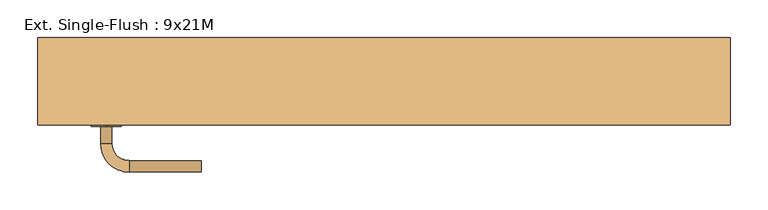
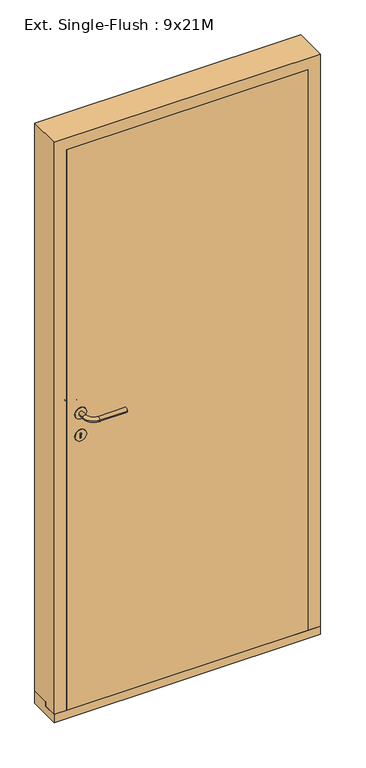
"""IFC4 building model written with IfcOpenShell, lengths in millimetres: door geometry, Ext. Single-Flush : 9x21M."""

import ifcopenshell
import ifcopenshell.guid

model = None  # the IFC model being written
_history = None  # IfcOwnerHistory: only IFC2X3 demands one
_inside = {}  # id of a spatial element -> (the spatial element, [elements in it])
_under = {}  # id of a project, library or spatial element -> (it, [spatial elements below it])
_declared = {}  # id of a project -> (the project, [libraries it declares])
_typed = {}  # id of a type object -> (the type object, [elements of that type])
_made_of = {}  # id of a material, layer set ... -> (it, [elements and type objects made of it])


def new_model(schema):
    """Start an empty IFC model of exactly this schema.

    Asked for "IFC4X3", IfcOpenShell would pick the latest addendum, in which some entities
    have other attributes; the version numbers below select the first issue.
    IFC2X3 requires an IfcOwnerHistory on every rooted entity: one is made here for all.
    """
    global model, _history
    if schema == "IFC4X3":
        model = ifcopenshell.file(schema_version=(4, 3, 0, 0))
    else:
        model = ifcopenshell.file(schema=schema)
    _inside.clear()
    _under.clear()
    _declared.clear()
    _typed.clear()
    _made_of.clear()
    _history = None
    if model.schema == "IFC2X3":
        org = make("IfcOrganization", Name="unknown")
        user = make(
            "IfcPersonAndOrganization",
            ThePerson=make("IfcPerson", FamilyName="unknown"),
            TheOrganization=org,
        )
        app = make(
            "IfcApplication",
            ApplicationDeveloper=org,
            Version="unknown",
            ApplicationFullName="unknown",
            ApplicationIdentifier="unknown",
        )
        _history = make(
            "IfcOwnerHistory",
            OwningUser=user,
            OwningApplication=app,
            ChangeAction="ADDED",
            CreationDate=0,
        )
    return model


def make(cls, **values):
    """One entity of the class cls with the attributes given. An attribute that is None is left unset."""
    return model.create_entity(
        cls, **{name: value for name, value in values.items() if value is not None}
    )


def rooted(cls, **values):
    """An entity with a GlobalId (a new one), such as an element, a storey or a relation."""
    return make(cls, GlobalId=ifcopenshell.guid.new(), OwnerHistory=_history, **values)


def si_unit(unit_type, name, prefix=None):
    """IfcSIUnit, for example si_unit("LENGTHUNIT", "METRE", prefix="MILLI")."""
    return make("IfcSIUnit", UnitType=unit_type, Prefix=prefix, Name=name)


def assignment(units):
    """IfcUnitAssignment: the units of a project."""
    return None if units is None else make("IfcUnitAssignment", Units=units)


def point(xyz):
    """IfcCartesianPoint."""
    return None if xyz is None else make("IfcCartesianPoint", Coordinates=xyz)


def direction(xyz):
    """IfcDirection."""
    return None if xyz is None else make("IfcDirection", DirectionRatios=xyz)


def frame(location, z_axis=None, x_axis=None):
    """IfcAxis2Placement3D, a coordinate frame: its origin and axes. An axis left out is left unset."""
    return make(
        "IfcAxis2Placement3D",
        Location=point(location),
        Axis=direction(z_axis),
        RefDirection=direction(x_axis),
    )


def frame_2d(location, x_axis=None):
    """IfcAxis2Placement2D, a coordinate frame in the plane: its origin and x axis."""
    return make(
        "IfcAxis2Placement2D", Location=point(location), RefDirection=direction(x_axis)
    )


def origin():
    """The frame at (0, 0, 0) with its axes left unset."""
    return frame((0.0, 0.0, 0.0))


def place(relative_to, where):
    """IfcLocalPlacement: puts the frame where relative to a parent placement (None: the world)."""
    return make(
        "IfcLocalPlacement", PlacementRelTo=relative_to, RelativePlacement=where
    )


def context(
    kind, dimensions, precision=None, world=None, true_north=None, identifier=None
):
    """IfcGeometricRepresentationContext, for example the 3D "Model" context."""
    return make(
        "IfcGeometricRepresentationContext",
        ContextIdentifier=identifier,
        ContextType=kind,
        CoordinateSpaceDimension=dimensions,
        Precision=precision,
        WorldCoordinateSystem=world,
        TrueNorth=true_north,
    )


def project(units=None, contexts=None):
    """IfcProject with its units and contexts."""
    return rooted(
        "IfcProject",
        Name="project",
        RepresentationContexts=contexts,
        UnitsInContext=assignment(units),
    )


def spatial(cls, under=None, at=None, **own):
    """A site, building, storey or space (cls), placed at a placement, below another one or the project."""
    s = rooted(cls, ObjectPlacement=at, **own)
    if under is not None:
        _under.setdefault(under.id(), (under, []))[1].append(s)
    return s


def polyline(points):
    """IfcPolyline through the points."""
    return make("IfcPolyline", Points=[point(p) for p in points])


def circle_curve(where, radius):
    """IfcCircle in the frame where."""
    return make("IfcCircle", Position=where, Radius=radius)


def ellipse_curve(where, semi_axis1, semi_axis2):
    """IfcEllipse in the frame where."""
    return make(
        "IfcEllipse", Position=where, SemiAxis1=semi_axis1, SemiAxis2=semi_axis2
    )


def trimmed(basis, trim1, trim2, sense, master):
    """IfcTrimmedCurve: the piece of a basis curve between two trims."""
    return make(
        "IfcTrimmedCurve",
        BasisCurve=basis,
        Trim1=trim1,
        Trim2=trim2,
        SenseAgreement=sense,
        MasterRepresentation=master,
    )


def segment(curve, same_sense, transition):
    """IfcCompositeCurveSegment."""
    return make(
        "IfcCompositeCurveSegment",
        Transition=transition,
        SameSense=same_sense,
        ParentCurve=curve,
    )


def composite_curve(segments, self_intersect=None):
    """IfcCompositeCurve: segments joined end to end."""
    return make("IfcCompositeCurve", Segments=segments, SelfIntersect=self_intersect)


def outline(outer, holes=None, kind="AREA"):
    """IfcArbitraryClosedProfileDef: a profile drawn as a closed curve; with holes, ...WithVoids."""
    if holes is None:
        return make("IfcArbitraryClosedProfileDef", ProfileType=kind, OuterCurve=outer)
    return make(
        "IfcArbitraryProfileDefWithVoids",
        ProfileType=kind,
        OuterCurve=outer,
        InnerCurves=holes,
    )


def extrude(swept, where, along, depth):
    """IfcExtrudedAreaSolid: the profile swept, set in the frame where, extruded along a direction by depth."""
    return make(
        "IfcExtrudedAreaSolid",
        SweptArea=swept,
        Position=where,
        ExtrudedDirection=direction(along),
        Depth=depth,
    )


def faces_of(points, faces, orient=None, outer=None):
    """IfcFace entities. A face is a list of loops; a loop is a list of indices into points, from 0.

    orient and outer hold one flag for each loop. By default every Orientation is true, the
    first loop of a face is its IfcFaceOuterBound and the others are IfcFaceBound.
    """
    made = []
    for i, loops in enumerate(faces):
        bounds = []
        for j, loop in enumerate(loops):
            is_outer = j == 0 if outer is None else outer[i][j]
            bounds.append(
                make(
                    "IfcFaceOuterBound" if is_outer else "IfcFaceBound",
                    Bound=make("IfcPolyLoop", Polygon=[points[k] for k in loop]),
                    Orientation=True if orient is None else orient[i][j],
                )
            )
        made.append(make("IfcFace", Bounds=bounds))
    return made


def faceted_brep(points, faces, orient=None, outer=None, voids=None):
    """IfcFacetedBrep: a solid bounded by flat faces; with voids (closed shells), ...WithVoids."""
    shared = [point(p) for p in points]
    hull = make("IfcClosedShell", CfsFaces=faces_of(shared, faces, orient, outer))
    if voids is None:
        return make("IfcFacetedBrep", Outer=hull)
    return make(
        "IfcFacetedBrepWithVoids",
        Outer=hull,
        Voids=[
            make(cls, CfsFaces=faces_of(shared, fs, o, b)) for cls, fs, o, b in voids
        ],
    )


def shape(context_of_items, identifier, shape_type, items):
    """IfcShapeRepresentation: the items that make up one representation, for example the "Body"."""
    return make(
        "IfcShapeRepresentation",
        ContextOfItems=context_of_items,
        RepresentationIdentifier=identifier,
        RepresentationType=shape_type,
        Items=items,
    )


def source(mapping_origin, context_of_items, identifier, shape_type, items):
    """IfcRepresentationMap: a shape defined once, which mapped items show again and again."""
    return make(
        "IfcRepresentationMap",
        MappingOrigin=mapping_origin,
        MappedRepresentation=shape(context_of_items, identifier, shape_type, items),
    )


def transform(
    local_origin,
    x_axis=None,
    y_axis=None,
    z_axis=None,
    scale=None,
    scale2=None,
    scale3=None,
    uniform=True,
):
    """IfcCartesianTransformationOperator3D, or its non-uniform kind. x_axis, y_axis, z_axis: its Axis1, 2, 3."""
    if uniform:
        return make(
            "IfcCartesianTransformationOperator3D",
            Axis1=direction(x_axis),
            Axis2=direction(y_axis),
            LocalOrigin=point(local_origin),
            Scale=scale,
            Axis3=direction(z_axis),
        )
    return make(
        "IfcCartesianTransformationOperator3DnonUniform",
        Axis1=direction(x_axis),
        Axis2=direction(y_axis),
        LocalOrigin=point(local_origin),
        Scale=scale,
        Axis3=direction(z_axis),
        Scale2=scale2,
        Scale3=scale3,
    )


def mapped(mapping_source, mapping_target):
    """IfcMappedItem: shows the shape of a source again, moved by a transform."""
    return make(
        "IfcMappedItem", MappingSource=mapping_source, MappingTarget=mapping_target
    )


def made_of(thing, what):
    """Note that an element or type object is made of a material, layer set ...; save() writes the relation."""
    if what is not None:
        _made_of.setdefault(what.id(), (what, []))[1].append(thing)
    return thing


def element(
    cls,
    number,
    at=None,
    inside=None,
    cuts=None,
    type_object=None,
    material=None,
    context=None,
    identifier="Body",
    shape_type=None,
    held_by="IfcProductDefinitionShape",
    body=None,
    shapes=None,
    **own,
):
    """One element of the class cls, such as IfcWall. Its Tag is "e" and its number.

    at: its placement. inside: the storey or other place that contains it. cuts: it is an
    opening in that element (IfcRelVoidsElement). A single representation is given by context,
    identifier, shape_type and body (its items); several are given by shapes. held_by: the class
    of the entity that holds the representations. save() writes the other relations.
    """
    e = rooted(cls, Tag="e%d" % number, ObjectPlacement=at, **own)
    if body is not None:
        shapes = [shape(context, identifier, shape_type, body)]
    if shapes is not None:
        e.Representation = make(held_by, Representations=shapes)
    if inside is not None:
        _inside.setdefault(inside.id(), (inside, []))[1].append(e)
    if cuts is not None:
        rooted(
            "IfcRelVoidsElement", RelatingBuildingElement=cuts, RelatedOpeningElement=e
        )
    if type_object is not None:
        _typed.setdefault(type_object.id(), (type_object, []))[1].append(e)
    return made_of(e, material)


def aggregate(whole, parts):
    """IfcRelAggregates: a whole, such as a stair, and the parts it consists of."""
    return rooted("IfcRelAggregates", RelatingObject=whole, RelatedObjects=parts)


def save(model, path):
    """Write the relations noted so far, then the file.

    IfcRelAggregates (storeys below a building ...), IfcRelContainedInSpatialStructure (elements
    in a storey), IfcRelDefinesByType, IfcRelAssociatesMaterial and IfcRelDeclares: one each for
    every whole, place, type object, material and project.
    """
    for whole, parts in _under.values():
        aggregate(whole, parts)
    for where, things in _inside.values():
        rooted(
            "IfcRelContainedInSpatialStructure",
            RelatedElements=things,
            RelatingStructure=where,
        )
    for kind, things in _typed.values():
        rooted("IfcRelDefinesByType", RelatedObjects=things, RelatingType=kind)
    for what, things in _made_of.values():
        rooted("IfcRelAssociatesMaterial", RelatedObjects=things, RelatingMaterial=what)
    for by, libraries in _declared.values():
        rooted("IfcRelDeclares", RelatingContext=by, RelatedDefinitions=libraries)
    model.write(path)


def plane_surface(at):
    """IfcPlane: the flat surface through the origin of the frame at, square to its z axis."""
    return make("IfcPlane", Position=at)


def cylinder_surface(at, radius):
    """IfcCylindricalSurface: all points at the distance radius from the z axis of the frame at."""
    return make("IfcCylindricalSurface", Position=at, Radius=radius)


def revolved_surface(curve, axis_point, axis_direction):
    """IfcSurfaceOfRevolution: the curve turned about the line through axis_point along axis_direction."""
    return make(
        "IfcSurfaceOfRevolution",
        SweptCurve=make("IfcArbitraryOpenProfileDef", ProfileType="CURVE", Curve=curve),
        AxisPosition=make("IfcAxis1Placement", Location=point(axis_point), Axis=direction(axis_direction)),
    )


def advanced_brep(points, edges, surfaces, faces):
    """IfcAdvancedBrep: a solid bounded by faces that lie on surfaces and meet in shared edges.

    An edge is (start, end): straight between two places in points (the first is 0);
    or (start, end, curve); or (start, end, curve, False) where it runs against its curve.
    A face is (place in surfaces, loops), or (place, loops, False) where it looks against
    its surface's normal. A loop lists edges by number (the first is 1), with a minus sign
    where the edge is run from its end to its start. The first loop is the outer one.
    """
    corners = [point(p) for p in points]
    vertices = [make("IfcVertexPoint", VertexGeometry=c) for c in corners]
    made = []
    for start, end, *more in edges:
        made.append(
            make(
                "IfcEdgeCurve",
                EdgeStart=vertices[start],
                EdgeEnd=vertices[end],
                EdgeGeometry=more[0] if more else make("IfcPolyline", Points=[corners[start], corners[end]]),
                SameSense=more[1] if len(more) > 1 else True,
            )
        )
    hull = []
    for where, loops, *sense in faces:
        bounds = []
        for j, loop in enumerate(loops):
            ring = [make("IfcOrientedEdge", EdgeElement=made[abs(k) - 1], Orientation=k > 0) for k in loop]
            bounds.append(
                make(
                    "IfcFaceOuterBound" if j == 0 else "IfcFaceBound",
                    Bound=make("IfcEdgeLoop", EdgeList=ring),
                    Orientation=True,
                )
            )
        hull.append(make("IfcAdvancedFace", Bounds=bounds, FaceSurface=surfaces[where], SameSense=sense[0] if sense else True))
    return make("IfcAdvancedBrep", Outer=make("IfcClosedShell", CfsFaces=hull))


def ext_single_flush_9x21m_ea871c4f(model_context):
    return source(origin(), model_context, "Body", "SolidModel", [
        extrude(outline(composite_curve([segment(trimmed(circle_curve(frame_2d((1090.0, -366.0)), 20.0), [point((1070.0, -366.0))], [point((1110.0, -366.0))], False, "CARTESIAN"), True, "CONTINUOUS"), segment(trimmed(circle_curve(frame_2d((1090.0, -366.0)), 20.0), [point((1110.0, -366.0))], [point((1070.0, -366.0))], False, "CARTESIAN"), True, "CONTINUOUS")], self_intersect=False)), frame((0.0, -186.0, 0.0), z_axis=(0.0, 1.0, 0.0), x_axis=(0.0, 0.0, 1.0)), (0.0, 0.0, 1.0), 2.0),
        advanced_brep(
        [(-373.5, -186.0, 1090.0), (-358.5, -186.0, 1090.0), (-358.5, -208.5, 1090.0), (-373.5, -208.5, 1090.0), (-336.0, -231.0, 1090.0), (-336.0, -246.0, 1090.0), (-241.0, -231.0, 1090.0), (-241.0, -246.0, 1090.0)],
        [
            (0, 1, circle_curve(frame((-366.0, -186.0, 1090.0), z_axis=(0.0, 1.0, 0.0), x_axis=(1.0, 0.0, 0.0)), 7.5)),
            (1, 0, circle_curve(frame((-366.0, -186.0, 1090.0), z_axis=(0.0, 1.0, 0.0), x_axis=(1.0, 0.0, 0.0)), 7.5)),
            (1, 2),
            (2, 3, circle_curve(frame((-366.0, -208.5, 1090.0), z_axis=(0.0, 1.0, 0.0), x_axis=(1.0, 0.0, 0.0)), 7.5)),
            (3, 0),
            (3, 2, circle_curve(frame((-366.0, -208.5, 1090.0), z_axis=(0.0, 1.0, 0.0), x_axis=(1.0, 0.0, 0.0)), 7.5)),
            (4, 5, circle_curve(frame((-336.0, -238.5, 1090.0), z_axis=(-1.0, 0.0, 0.0), x_axis=(0.0, 1.0, 0.0)), 7.5)),
            (5, 3, circle_curve(frame((-336.0, -208.5, 1090.0), z_axis=(0.0, 0.0, -1.0), x_axis=(-1.0, 0.0, 0.0)), 37.5)),
            (2, 4, circle_curve(frame((-336.0, -208.5, 1090.0), z_axis=(0.0, 0.0, 1.0), x_axis=(-1.0, 0.0, 0.0)), 22.5)),
            (5, 4, circle_curve(frame((-336.0, -238.5, 1090.0), z_axis=(-1.0, 0.0, 0.0), x_axis=(0.0, 1.0, 0.0)), 7.5)),
            (4, 6),
            (6, 7, circle_curve(frame((-241.0, -238.5, 1090.0), z_axis=(-1.0, 0.0, 0.0), x_axis=(0.0, 1.0, 0.0)), 7.5)),
            (7, 5),
            (7, 6, circle_curve(frame((-241.0, -238.5, 1090.0), z_axis=(-1.0, 0.0, 0.0), x_axis=(0.0, 1.0, 0.0)), 7.5)),
        ],
        [
            plane_surface(frame((-366.0, -186.0, 1090.0), z_axis=(0.0, 1.0, 0.0), x_axis=(0.0, 0.0, -1.0))),
            cylinder_surface(frame((-366.0, -186.0, 1090.0), z_axis=(0.0, 1.0, 0.0), x_axis=(1.0, 0.0, 0.0)), 7.5),
            revolved_surface(trimmed(ellipse_curve(frame((-366.0, -208.5, 1090.0), z_axis=(0.0, -1.0, 0.0), x_axis=(1.0, 0.0, 0.0)), 7.5, 7.5), [point((-373.5, -208.5, 1090.0))], [point((-358.5, -208.5, 1090.0))], True, "CARTESIAN"), (-336.0, -208.5, 1090.0), (0.0, 0.0, -1.0)),
            revolved_surface(trimmed(ellipse_curve(frame((-366.0, -208.5, 1090.0), z_axis=(0.0, -1.0, 0.0), x_axis=(1.0, 0.0, 0.0)), 7.5, 7.5), [point((-358.5, -208.5, 1090.0))], [point((-373.5, -208.5, 1090.0))], True, "CARTESIAN"), (-336.0, -208.5, 1090.0), (0.0, 0.0, -1.0)),
            cylinder_surface(frame((-336.0, -238.5, 1090.0), z_axis=(-1.0, 0.0, 0.0), x_axis=(0.0, 1.0, 0.0)), 7.5),
            plane_surface(frame((-241.0, -238.5, 1090.0), z_axis=(1.0, 0.0, 0.0), x_axis=(0.0, 0.0, -1.0))),
        ],
        [
            (0, [[1, 2]]),
            (1, [[3, 4, 5, -2]]),
            (1, [[-5, 6, -3, -1]]),
            (2, [[7, 8, -4, 9]]),
            (3, [[10, -9, -6, -8]]),
            (4, [[11, 12, 13, -7]]),
            (4, [[-13, 14, -11, -10]]),
            (5, [[-12, -14]]),
        ],
    ),
        extrude(outline(composite_curve([segment(trimmed(circle_curve(frame_2d((1010.0, -366.0)), 20.0), [point((990.0, -366.0))], [point((1030.0, -366.0))], False, "CARTESIAN"), True, "CONTINUOUS"), segment(trimmed(circle_curve(frame_2d((1010.0, -366.0)), 20.0), [point((1030.0, -366.0))], [point((990.0, -366.0))], False, "CARTESIAN"), True, "CONTINUOUS")], self_intersect=False), holes=[composite_curve([segment(trimmed(circle_curve(frame_2d((1015.0, -366.0)), 3.0), [point((1012.4019238, -367.5))], [point((1012.4019238, -364.5))], True, "CARTESIAN"), True, "CONTINUOUS"), segment(polyline([(1012.4019238, -364.5), (1000.0, -364.5), (1000.0, -367.5), (1012.4019238, -367.5)]), True, "CONTINUOUS")], self_intersect=False)]), frame((0.0, -186.0, 0.0), z_axis=(0.0, 1.0, 0.0), x_axis=(0.0, 0.0, 1.0)), (0.0, 0.0, 1.0), 2.0),
        extrude(outline(composite_curve([segment(trimmed(circle_curve(frame_2d((1090.0, -366.0)), 20.0), [point((1070.0, -366.0))], [point((1110.0, -366.0))], False, "CARTESIAN"), True, "CONTINUOUS"), segment(trimmed(circle_curve(frame_2d((1090.0, -366.0)), 20.0), [point((1110.0, -366.0))], [point((1070.0, -366.0))], False, "CARTESIAN"), True, "CONTINUOUS")], self_intersect=False)), frame((0.0, -134.0, 0.0), z_axis=(0.0, 1.0, 0.0), x_axis=(0.0, 0.0, 1.0)), (0.0, 0.0, 1.0), 2.0),
        advanced_brep(
        [(-373.5, -132.0, 1090.0), (-358.5, -132.0, 1090.0), (-373.5, -109.5, 1090.0), (-358.5, -109.5, 1090.0), (-336.0, -87.0, 1090.0), (-336.0, -72.0, 1090.0), (-241.0, -72.0, 1090.0), (-241.0, -87.0, 1090.0)],
        [
            (0, 1, circle_curve(frame((-366.0, -132.0, 1090.0), z_axis=(0.0, -1.0, 0.0), x_axis=(1.0, 0.0, 0.0)), 7.5)),
            (1, 0, circle_curve(frame((-366.0, -132.0, 1090.0), z_axis=(0.0, -1.0, 0.0), x_axis=(1.0, 0.0, 0.0)), 7.5)),
            (0, 2),
            (2, 3, circle_curve(frame((-366.0, -109.5, 1090.0), z_axis=(0.0, -1.0, 0.0), x_axis=(1.0, 0.0, 0.0)), 7.5)),
            (3, 1),
            (3, 2, circle_curve(frame((-366.0, -109.5, 1090.0), z_axis=(0.0, -1.0, 0.0), x_axis=(1.0, 0.0, 0.0)), 7.5)),
            (4, 3, circle_curve(frame((-336.0, -109.5, 1090.0), z_axis=(0.0, 0.0, 1.0), x_axis=(-1.0, 0.0, 0.0)), 22.5)),
            (2, 5, circle_curve(frame((-336.0, -109.5, 1090.0), z_axis=(0.0, 0.0, -1.0), x_axis=(-1.0, 0.0, 0.0)), 37.5)),
            (5, 4, circle_curve(frame((-336.0, -79.5, 1090.0), z_axis=(-1.0, 0.0, 0.0), x_axis=(0.0, -1.0, 0.0)), 7.5)),
            (4, 5, circle_curve(frame((-336.0, -79.5, 1090.0), z_axis=(-1.0, 0.0, 0.0), x_axis=(0.0, -1.0, 0.0)), 7.5)),
            (5, 6),
            (6, 7, circle_curve(frame((-241.0, -79.5, 1090.0), z_axis=(-1.0, 0.0, 0.0), x_axis=(0.0, -1.0, 0.0)), 7.5)),
            (7, 4),
            (7, 6, circle_curve(frame((-241.0, -79.5, 1090.0), z_axis=(-1.0, 0.0, 0.0), x_axis=(0.0, -1.0, 0.0)), 7.5)),
        ],
        [
            plane_surface(frame((-366.0, -132.0, 1090.0), z_axis=(0.0, -1.0, 0.0), x_axis=(0.0, 0.0, -1.0))),
            cylinder_surface(frame((-366.0, -132.0, 1090.0), z_axis=(0.0, -1.0, 0.0), x_axis=(1.0, 0.0, 0.0)), 7.5),
            revolved_surface(trimmed(ellipse_curve(frame((-366.0, -109.5, 1090.0), z_axis=(0.0, -1.0, 0.0), x_axis=(1.0, 0.0, 0.0)), 7.5, 7.5), [point((-373.5, -109.5, 1090.0))], [point((-358.5, -109.5, 1090.0))], True, "CARTESIAN"), (-336.0, -109.5, 1090.0), (0.0, 0.0, -1.0)),
            revolved_surface(trimmed(ellipse_curve(frame((-366.0, -109.5, 1090.0), z_axis=(0.0, -1.0, 0.0), x_axis=(1.0, 0.0, 0.0)), 7.5, 7.5), [point((-358.5, -109.5, 1090.0))], [point((-373.5, -109.5, 1090.0))], True, "CARTESIAN"), (-336.0, -109.5, 1090.0), (0.0, 0.0, -1.0)),
            cylinder_surface(frame((-336.0, -79.5, 1090.0), z_axis=(-1.0, 0.0, 0.0), x_axis=(0.0, -1.0, 0.0)), 7.5),
            plane_surface(frame((-241.0, -79.5, 1090.0), z_axis=(1.0, 0.0, 0.0), x_axis=(0.0, 0.0, -1.0))),
        ],
        [
            (0, [[1, 2]]),
            (1, [[-1, 3, 4, 5]]),
            (1, [[-2, -5, 6, -3]]),
            (2, [[7, -4, 8, 9]]),
            (3, [[-8, -6, -7, 10]]),
            (4, [[-9, 11, 12, 13]]),
            (4, [[-10, -13, 14, -11]]),
            (5, [[-14, -12]]),
        ],
    ),
        extrude(outline(composite_curve([segment(trimmed(circle_curve(frame_2d((1010.0, -366.0)), 20.0), [point((990.0, -366.0))], [point((1030.0, -366.0))], False, "CARTESIAN"), True, "CONTINUOUS"), segment(trimmed(circle_curve(frame_2d((1010.0, -366.0)), 20.0), [point((1030.0, -366.0))], [point((990.0, -366.0))], False, "CARTESIAN"), True, "CONTINUOUS")], self_intersect=False), holes=[composite_curve([segment(trimmed(circle_curve(frame_2d((1015.0, -366.0)), 3.0), [point((1012.4019238, -367.5))], [point((1012.4019238, -364.5))], True, "CARTESIAN"), True, "CONTINUOUS"), segment(polyline([(1012.4019238, -364.5), (1000.0, -364.5), (1000.0, -367.5), (1012.4019238, -367.5)]), True, "CONTINUOUS")], self_intersect=False)]), frame((0.0, -134.0, 0.0), z_axis=(0.0, 1.0, 0.0), x_axis=(0.0, 0.0, 1.0)), (0.0, 0.0, 1.0), 2.0),
        extrude(outline(polyline([(-414.0, -184.0), (-414.0, -134.0), (414.0, -134.0), (414.0, -184.0), (-414.0, -184.0)])), frame((0.0, 0.0, 30.0), z_axis=(0.0, 0.0, 1.0), x_axis=(1.0, 0.0, 0.0)), (0.0, 0.0, 1.0), 2028.0),
        faceted_brep([(414.0, -184.0, 2058.0), (414.0, -184.0, 30.0), (456.0, -184.0, 30.0), (456.0, -184.0, 2100.0), (-456.0, -184.0, 2100.0), (-456.0, -184.0, 30.0), (-414.0, -184.0, 30.0), (-414.0, -184.0, 2058.0), (-414.0, -134.0, 30.0), (-414.0, -134.0, 45.0), (-414.0, -134.0, 2058.0), (-456.0, -134.0, 30.0), (456.0, -134.0, 30.0), (414.0, -134.0, 30.0), (-456.0, -69.0, 2100.0), (-456.0, -69.0, 45.0), (-456.0, -134.0, 45.0), (456.0, -134.0, 45.0), (456.0, -69.0, 45.0), (456.0, -69.0, 2100.0), (414.0, -134.0, 2058.0), (414.0, -134.0, 45.0), (399.0, -69.0, 45.0), (399.0, -69.0, 2043.0), (-399.0, -69.0, 2043.0), (-399.0, -69.0, 45.0), (-399.0, -134.0, 45.0), (399.0, -134.0, 45.0), (-399.0, -134.0, 2043.0), (399.0, -134.0, 2043.0)], [[[0, 1, 2, 3, 4, 5, 6, 7]], [[7, 6, 8, 9, 10]], [[8, 6, 5, 11]], [[12, 2, 1, 13]], [[14, 15, 16, 11, 5, 4]], [[3, 2, 12, 17, 18, 19]], [[20, 21, 13, 1, 0]], [[19, 18, 22, 23, 24, 25, 15, 14]], [[16, 15, 25, 26, 9]], [[21, 27, 22, 18, 17]], [[9, 8, 11, 16]], [[17, 12, 13, 21]], [[28, 26, 25, 24]], [[23, 22, 27, 29]], [[29, 27, 21, 20, 10, 9, 26, 28]], [[3, 19, 14, 4]], [[23, 29, 28, 24]], [[7, 10, 20, 0]]]),
        extrude(outline(polyline([(-184.0, 30.0), (-134.0, 30.0), (-134.0, 45.0), (-69.0, 45.0), (-69.0, 0.0), (-184.0, 0.0), (-184.0, 30.0)])), frame((-456.0, 0.0, 0.0), z_axis=(1.0, 0.0, 0.0), x_axis=(0.0, 1.0, 0.0)), (0.0, 0.0, 1.0), 912.0),
    ])


if __name__ == "__main__":
    model = new_model("IFC4")
    model_context = context("Model", 3, world=origin())
    ifc_project = project(units=[si_unit("LENGTHUNIT", "METRE", prefix="MILLI")], contexts=[model_context])
    site = spatial("IfcSite", under=ifc_project)
    building = spatial("IfcBuilding", under=site)
    placement = place(None, origin())
    ext_single_flush_9x21m_shape = ext_single_flush_9x21m_ea871c4f(model_context)
    element("IfcDoor", 1, ObjectType="Ext. Single-Flush : 9x21M", at=placement, inside=building, context=model_context, shape_type="MappedRepresentation", body=[
        mapped(ext_single_flush_9x21m_shape, transform((0.0, 0.0, 0.0), x_axis=(1.0, 0.0, 0.0), y_axis=(0.0, 1.0, 0.0), z_axis=(0.0, 0.0, 1.0))),
    ])
    save(model, "model.ifc")

# Revit data of these elements
# Project information
#   Client Name = "Test Project"
#   Project Address = "Enter address here"
#   Project Number = "Number"
#   Current Version = "0.0.0"
#   SR Document GUID = "3eb9317e-835d-4f79-8926-4d15b96bc824"
# Type "Ext. Single-Flush : 9x21M"
#   Type Mark = "51"
#   Sound Rating = ""
#   Opening Side [instance default] = ""
#   Hinge Side [instance default] = ""
#   Creator Organization [instance default] = "© Danish Educational Content"
#   Creator Name [instance default] = "© Erik Falck Jørgensen"
#   Creator Build [instance default] = "2017.0301.0"
#   Analytic Construction = "<None>"
#   length#6 = -50 mm
#   length#5 = 912 mm
#   length#4 = 120 mm
#   length#3 = 30 mm
#   length#2 = 57 mm
#   length#1 = 0 mm
#   Thickness = 50 mm
#   Seal Width = 12 mm
#   Rough Width = 912 mm
#   Rough Height = 2100 mm
#   Rebate Depth = 50 mm
#   Rabbet Width = 15 mm
#   Rabbet Depth = 50 mm
#   Height = 2088 mm
#   Width = 888 mm
#   Handle From Side = 90 mm
#   Handle From Bottom = 1090 mm
#   Exterior Direction [instance default] = 0.00°
#   Case Width = 45 mm
#   Case Depth = 115 mm
#   Threshold = yes
#   Sealing = no
#   Hinging = yes
#   Wall Closure = 1
#   Function = 1
#   Panel = none
#   Handle Finish = none
#   Handle = element 507533
#   Embrasure Interior = none
#   Embrasure Exterior = none
#   Case/Transom = none
#   Assembly Code = ""
# Element 1 (IfcDoor, "Ext. Single-Flush : 9x21M")
#   Materials on its faces: "Stainless Steel, Polished", "Default Frame/Mullion (Interior/Exterior)", "Default Door Panel (Exterior/Interior)"
# Materials
#   "Stainless Steel, Polished": class "Metal", colour RGB 180 180 180, transparency 0, Description = "Rustfri stål, poleret", Cost = 0
#   "Default Frame/Mullion (Interior/Exterior)": class "Generic", colour RGB 205 205 205, transparency 0, Description = "Udefineret karm/ramme materiale", Cost = 0
#   "Default Door Panel (Exterior/Interior)": class "Generic", colour RGB 205 205 205, transparency 0, Description = "Udefineret dørplade materiale", Cost = 0
